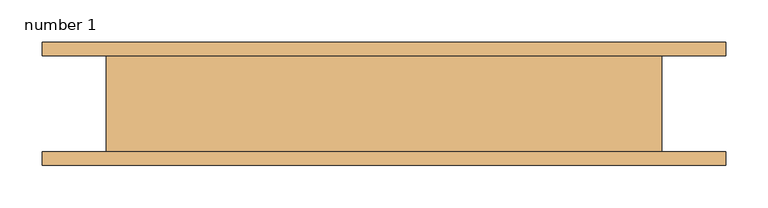
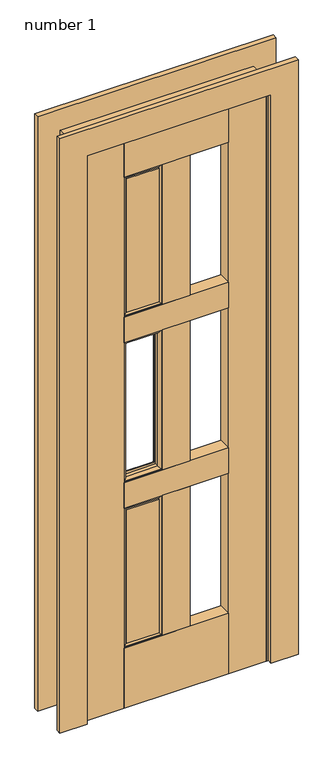
"""IFC4 building model written with IfcOpenShell, lengths in millimetres: door geometry, Door-Interior-Karona-K5660-6_Panel : number 1."""

from ifc_helpers import new_model, si_unit, frame, origin, origin_with_axes, place, context, project, spatial, polyline, ellipse_curve, outline, extrude, faceted_brep, source, transform, mapped, element, save
from ifc_brep_helpers import plane_surface, cylinder_surface, revolved_surface, advanced_brep


def number_1_f33ada90(model_context):
    return source(origin(), model_context, "Body", "SolidModel", [
        advanced_brep(
        [(-177.8, -15.2908, 1311.275), (-46.0375, -15.2908, 1311.275), (-57.3628137, -24.6126, 1299.9496863), (-166.4746863, -24.6126, 1299.9496863), (-57.1627, -46.3324899, 1300.1498), (-57.1627, -46.3324899, 820.7502), (-48.2727, -54.4576, 811.8602), (-48.2727, -54.4576, 1309.0398), (-166.6748, -46.3324899, 820.7502), (-166.6748, -46.3324899, 1300.1498), (-175.5648, -54.4576, 1309.0398), (-175.5648, -54.4576, 811.8602), (-46.0375, -54.4576, 809.625), (-177.8, -54.4576, 809.625), (-177.8, -15.2908, 809.625), (-46.0375, -15.2908, 809.625), (-57.1627, -34.7218, 820.7502), (-166.6748, -34.7218, 820.7502), (-47.3075, -24.6126, 1310.005), (-47.3075, -24.6126, 810.895), (-47.3075, -34.7218, 810.895), (-47.3075, -34.7218, 1310.005), (-176.53, -24.6126, 810.895), (-176.53, -24.6126, 1310.005), (-57.3628137, -24.6126, 820.9503137), (-166.4746863, -24.6126, 820.9503137), (-176.53, -34.7218, 810.895), (-177.8, -54.4576, 1311.275), (-166.6748, -34.7218, 1300.1498), (-176.53, -34.7218, 1310.005), (-46.0375, -54.4576, 1311.275), (-57.1627, -34.7218, 1300.1498)],
        [
            (0, 1),
            (1, 2, ellipse_curve(frame((-47.0685124, -25.5788135, 1310.2439876), z_axis=(-0.7071067811865475, 0.0, 0.7071067811865475), x_axis=(-0.7071067811865476, 0.0, -0.7071067811865474)), 14.6223259, 10.3395458)),
            (2, 3),
            (3, 0, ellipse_curve(frame((-176.7689876, -25.5788135, 1310.2439876), z_axis=(0.7071067811865475, 0.0, 0.7071067811865475), x_axis=(-0.7071067811865476, 0.0, 0.7071067811865474)), 14.6223259, 10.3395458)),
            (4, 5),
            (5, 6, ellipse_curve(frame((-48.2727, -45.531597, 811.8602), z_axis=(0.7071067811865475, 0.0, 0.7071067811865475), x_axis=(-0.7071067811865474, 0.0, 0.7071067811865476)), 12.6232745, 8.926003)),
            (6, 7),
            (7, 4, ellipse_curve(frame((-48.2727, -45.531597, 1309.0398), z_axis=(0.7071067811865475, 0.0, -0.7071067811865475), x_axis=(0.7071067811865474, 0.0, 0.7071067811865476)), 12.6232745, 8.926003)),
            (8, 9),
            (9, 10, ellipse_curve(frame((-175.5648, -45.531597, 1309.0398), z_axis=(-0.7071067811865475, 0.0, -0.7071067811865475), x_axis=(0.7071067811865474, 0.0, -0.7071067811865476)), 12.6232745, 8.926003)),
            (10, 11),
            (11, 8, ellipse_curve(frame((-175.5648, -45.531597, 811.8602), z_axis=(-0.7071067811865475, 0.0, 0.7071067811865475), x_axis=(-0.7071067811865474, 0.0, -0.7071067811865476)), 12.6232745, 8.926003)),
            (12, 13),
            (13, 14),
            (14, 15),
            (15, 12),
            (16, 17),
            (17, 8),
            (8, 5),
            (5, 16),
            (18, 19),
            (19, 20),
            (20, 21),
            (21, 18),
            (22, 19),
            (18, 23),
            (23, 22),
            (24, 25),
            (25, 3),
            (2, 24),
            (14, 25, ellipse_curve(frame((-176.7689876, -25.5788135, 810.6560124), z_axis=(0.7071067811865475, 0.0, -0.7071067811865475), x_axis=(0.7071067811865476, 0.0, 0.7071067811865474)), 14.6223259, 10.3395458)),
            (24, 15, ellipse_curve(frame((-47.0685124, -25.5788135, 810.6560124), z_axis=(-0.7071067811865475, 0.0, -0.7071067811865475), x_axis=(0.7071067811865476, 0.0, -0.7071067811865474)), 14.6223259, 10.3395458)),
            (22, 26),
            (26, 20),
            (13, 27),
            (27, 0),
            (0, 14),
            (17, 28),
            (28, 9),
            (23, 29),
            (29, 26),
            (27, 30),
            (30, 1),
            (28, 31),
            (31, 4),
            (4, 9),
            (21, 29),
            (30, 12),
            (15, 1),
            (31, 16),
            (6, 11),
            (10, 7),
        ],
        [
            cylinder_surface(frame((-177.8, -25.5788135, 1310.2439876), z_axis=(-1.0, 0.0, 0.0), x_axis=(0.0, 1.0, 0.0)), 10.3395458),
            cylinder_surface(frame((-48.2727, -45.531597, 1311.275), z_axis=(0.0, 0.0, 1.0), x_axis=(0.0, 1.0, 0.0)), 8.926003),
            cylinder_surface(frame((-175.5648, -45.531597, 809.625), z_axis=(0.0, 0.0, -1.0), x_axis=(0.0, 1.0, 0.0)), 8.926003),
            plane_surface(frame((-46.0375, -15.2908, 809.625), z_axis=(0.0, 0.0, -1.0), x_axis=(-1.0, 0.0, 0.0))),
            plane_surface(frame((-57.1627, -46.3324899, 820.7502), z_axis=(0.0, 0.0, 1.0), x_axis=(-1.0, 0.0, 0.0))),
            plane_surface(frame((-47.3075, -34.7218, 1310.005), z_axis=(-1.0, 0.0, 0.0), x_axis=(0.0, 0.0, -1.0))),
            plane_surface(frame((-47.3075, -24.6126, 1310.005), z_axis=(0.0, -1.0, 0.0), x_axis=(0.0, 0.0, -1.0))),
            cylinder_surface(frame((-46.0375, -25.5788135, 810.6560124), z_axis=(1.0, 0.0, 0.0), x_axis=(0.0, 1.0, 0.0)), 10.3395458),
            plane_surface(frame((-47.3075, -34.7218, 810.895), z_axis=(0.0, 0.0, 1.0), x_axis=(-1.0, 0.0, 0.0))),
            plane_surface(frame((-177.8, -15.2908, 809.625), z_axis=(-1.0, 0.0, 0.0), x_axis=(0.0, 0.0, 1.0))),
            plane_surface(frame((-166.6748, -46.3324899, 820.7502), z_axis=(1.0, 0.0, 0.0), x_axis=(0.0, 0.0, 1.0))),
            plane_surface(frame((-176.53, -34.7218, 810.895), z_axis=(1.0, 0.0, 0.0), x_axis=(0.0, 0.0, 1.0))),
            plane_surface(frame((-177.8, -15.2908, 1311.275), z_axis=(0.0, 0.0, 1.0), x_axis=(1.0, 0.0, 0.0))),
            plane_surface(frame((-166.6748, -46.3324899, 1300.1498), z_axis=(0.0, 0.0, -1.0), x_axis=(1.0, 0.0, 0.0))),
            plane_surface(frame((-176.53, -34.7218, 1310.005), z_axis=(0.0, 0.0, -1.0), x_axis=(1.0, 0.0, 0.0))),
            plane_surface(frame((-46.0375, -15.2908, 1311.275), z_axis=(1.0, 0.0, 0.0), x_axis=(0.0, 0.0, -1.0))),
            plane_surface(frame((-57.1627, -46.3324899, 1300.1498), z_axis=(-1.0, 0.0, 0.0), x_axis=(0.0, 0.0, -1.0))),
            plane_surface(frame((-57.1627, -34.7218, 1300.1498), z_axis=(0.0, 1.0, 0.0), x_axis=(0.0, 0.0, -1.0))),
            plane_surface(frame((-46.0375, -54.4576, 1311.275), z_axis=(0.0, -1.0, 0.0), x_axis=(0.0, 0.0, -1.0))),
            cylinder_surface(frame((-46.0375, -45.531597, 811.8602), z_axis=(1.0, 0.0, 0.0), x_axis=(0.0, 1.0, 0.0)), 8.926003),
            cylinder_surface(frame((-176.7689876, -25.5788135, 809.625), z_axis=(0.0, 0.0, -1.0), x_axis=(0.0, 1.0, 0.0)), 10.3395458),
            cylinder_surface(frame((-177.8, -45.531597, 1309.0398), z_axis=(-1.0, 0.0, 0.0), x_axis=(0.0, 1.0, 0.0)), 8.926003),
            cylinder_surface(frame((-47.0685124, -25.5788135, 1311.275), z_axis=(0.0, 0.0, 1.0), x_axis=(0.0, 1.0, 0.0)), 10.3395458),
        ],
        [
            (0, [[1, 2, 3, 4]]),
            (1, [[5, 6, 7, 8]]),
            (2, [[9, 10, 11, 12]]),
            (3, [[13, 14, 15, 16]]),
            (4, [[17, 18, 19, 20]]),
            (5, [[21, 22, 23, 24]]),
            (6, [[25, -21, 26, 27], [28, 29, -3, 30]]),
            (7, [[-15, 31, -28, 32]]),
            (8, [[-25, 33, 34, -22]]),
            (9, [[35, 36, 37, -14]]),
            (10, [[38, 39, -9, -18]]),
            (11, [[-27, 40, 41, -33]]),
            (12, [[42, 43, -1, -36]]),
            (13, [[44, 45, 46, -39]]),
            (14, [[-26, -24, 47, -40]]),
            (15, [[48, -16, 49, -43]]),
            (16, [[50, -20, -5, -45]]),
            (17, [[-34, -41, -47, -23], [-17, -50, -44, -38]]),
            (18, [[-13, -48, -42, -35], [51, -11, 52, -7]]),
            (19, [[-19, -12, -51, -6]]),
            (20, [[-37, -4, -29, -31]]),
            (21, [[-46, -8, -52, -10]]),
            (22, [[-49, -32, -30, -2]]),
        ],
    ),
        advanced_brep(
        [(-166.6748, -54.4576, 1893.8748), (-166.6748, -54.4576, 1414.4752), (-57.1627, -54.4576, 1414.4752), (-57.1627, -54.4576, 1893.8748), (-166.6748, -34.7218, 1893.8748), (-166.6748, -36.0454899, 1893.8748), (-57.1627, -36.0454899, 1893.8748), (-57.1627, -34.7218, 1893.8748), (-57.1627, -44.5515929, 1893.8748), (-166.6748, -44.5515929, 1893.8748), (-57.1627, -34.7218, 1414.4752), (-57.1627, -36.0454899, 1414.4752), (-166.6748, -36.0454899, 1414.4752), (-166.6748, -34.7218, 1414.4752), (-166.6748, -44.5515929, 1414.4752), (-57.1627, -44.5515929, 1414.4752), (-87.1686653, -44.5515929, 1863.8688347), (-136.6688347, -44.5515929, 1863.8688347), (-87.1686653, -44.5515929, 1444.4811653), (-136.6688347, -44.5515929, 1444.4811653)],
        [
            (0, 1),
            (1, 2),
            (2, 3),
            (3, 0),
            (4, 5),
            (5, 6),
            (6, 7),
            (7, 4),
            (3, 8),
            (8, 9),
            (9, 0),
            (10, 11),
            (11, 12),
            (12, 13),
            (13, 10),
            (1, 14),
            (14, 15),
            (15, 2),
            (9, 14),
            (12, 5),
            (4, 13),
            (6, 11),
            (10, 7),
            (15, 8),
            (16, 6, ellipse_curve(frame((-55.2243315, -100.0605261, 1895.8131685), z_axis=(0.7071067811865475, 0.0, -0.7071067811865475), x_axis=(-0.7071067811865476, 0.0, -0.7071067811865474)), 90.5724254, 64.0443762)),
            (5, 17, ellipse_curve(frame((-168.6131685, -100.0605261, 1895.8131685), z_axis=(-0.7071067811865475, 0.0, -0.7071067811865475), x_axis=(-0.7071067811865476, 0.0, 0.7071067811865474)), 90.5724254, 64.0443762)),
            (17, 16),
            (18, 11, ellipse_curve(frame((-55.2243315, -100.0605261, 1412.5368315), z_axis=(-0.7071067811865475, 0.0, -0.7071067811865475), x_axis=(-0.7071067811865474, 0.0, 0.7071067811865476)), 90.5724254, 64.0443762)),
            (16, 18),
            (19, 12, ellipse_curve(frame((-168.6131685, -100.0605261, 1412.5368315), z_axis=(-0.7071067811865475, 0.0, 0.7071067811865475), x_axis=(0.7071067811865476, 0.0, 0.7071067811865474)), 90.5724254, 64.0443762)),
            (18, 19),
            (19, 17),
        ],
        [
            plane_surface(frame((-57.1627, -54.4576, 1893.8748), z_axis=(0.0, -1.0, 0.0), x_axis=(0.0, 0.0, -1.0))),
            plane_surface(frame((-57.1627, -34.7218, 1893.8748), z_axis=(0.0, 0.0, 1.0), x_axis=(1.0, 0.0, 0.0))),
            plane_surface(frame((-57.1627, -34.7218, 1414.4752), z_axis=(0.0, 0.0, -1.0), x_axis=(-1.0, 0.0, 0.0))),
            plane_surface(frame((-166.6748, -54.4576, 1893.8748), z_axis=(-1.0, 0.0, 0.0), x_axis=(0.0, 0.0, -1.0))),
            plane_surface(frame((-57.1627, -34.7218, 1893.8748), z_axis=(1.0, 0.0, 0.0), x_axis=(0.0, 0.0, -1.0))),
            plane_surface(frame((-166.6748, -34.7218, 1893.8748), z_axis=(0.0, 1.0, 0.0), x_axis=(0.0, 0.0, -1.0))),
            revolved_surface(polyline([(-232.6575446888527, -100.0605261, 1831.7687923), (8.820044688852704, -100.0605261, 1831.7687923)]), (-177.8, -100.0605261, 1895.8131685), (-1.0, 0.0, 0.0)),
            revolved_surface(polyline([(-119.2687077, -100.0605261, 1959.8575446888528), (-119.2687077, -100.0605261, 1348.4924553111473)]), (-55.2243315, -100.0605261, 1905.0), (0.0, 0.0, 1.0)),
            revolved_surface(polyline([(8.820044688852683, -100.0605261, 1476.5812077), (-232.6575446888527, -100.0605261, 1476.5812077)]), (-46.0375, -100.0605261, 1412.5368315), (1.0, 0.0, 0.0)),
            revolved_surface(polyline([(-104.5687923, -100.0605261, 1348.4924553111473), (-104.5687923, -100.0605261, 1959.8575446888526)]), (-168.6131685, -100.0605261, 1403.35), (0.0, 0.0, -1.0)),
            plane_surface(frame((-177.8, -44.5515929, 1403.35), z_axis=(0.0, 1.0, 0.0), x_axis=(0.0, 0.0, 1.0))),
        ],
        [
            (0, [[1, 2, 3, 4]]),
            (1, [[5, 6, 7, 8]]),
            (1, [[9, 10, 11, -4]]),
            (2, [[12, 13, 14, 15]]),
            (2, [[16, 17, 18, -2]]),
            (3, [[-11, 19, -16, -1]]),
            (3, [[-14, 20, -5, 21]]),
            (4, [[-7, 22, -12, 23]]),
            (4, [[-18, 24, -9, -3]]),
            (5, [[-23, -15, -21, -8]]),
            (6, [[25, -6, 26, 27]]),
            (7, [[28, -22, -25, 29]]),
            (8, [[30, -13, -28, 31]]),
            (9, [[-26, -20, -30, 32]]),
            (10, [[-24, -17, -19, -10], [-32, -31, -29, -27]]),
        ],
    ),
        advanced_brep(
        [(-166.6748, -24.6126, 1893.8748), (-166.6748, -24.6126, 1414.4752), (-57.1627, -24.6126, 1414.4752), (-57.1627, -24.6126, 1893.8748), (-137.8448579, -15.4432, 1443.3051421), (-137.8448579, -15.4432, 1865.0448579), (-85.9926421, -15.4432, 1865.0448579), (-85.9926421, -15.4432, 1443.3051421), (-57.1627, -23.2889101, 1893.8748), (-166.6748, -23.2889101, 1893.8748), (-166.6748, -23.2889101, 1414.4752), (-57.1627, -23.2889101, 1414.4752)],
        [
            (0, 1),
            (1, 2),
            (2, 3),
            (3, 0),
            (4, 5),
            (5, 6),
            (6, 7),
            (7, 4),
            (3, 8),
            (8, 9),
            (9, 0),
            (1, 10),
            (10, 11),
            (11, 2),
            (7, 11, ellipse_curve(frame((-55.2243315, 40.7261261, 1412.5368315), z_axis=(0.7071067811865475, 0.0, 0.7071067811865475), x_axis=(0.7071067811865476, 0.0, -0.7071067811865474)), 90.5724254, 64.0443762)),
            (10, 4, ellipse_curve(frame((-168.6131685, 40.7261261, 1412.5368315), z_axis=(-0.7071067811865475, 0.0, 0.7071067811865475), x_axis=(0.7071067811865476, 0.0, 0.7071067811865474)), 90.5724254, 64.0443762)),
            (10, 9),
            (9, 5, ellipse_curve(frame((-168.6131685, 40.7261261, 1895.8131685), z_axis=(0.7071067811865475, 0.0, 0.7071067811865475), x_axis=(0.7071067811865474, 0.0, -0.7071067811865476)), 90.5724254, 64.0443762)),
            (8, 6, ellipse_curve(frame((-55.2243315, 40.7261261, 1895.8131685), z_axis=(0.7071067811865475, 0.0, -0.7071067811865475), x_axis=(-0.7071067811865476, 0.0, -0.7071067811865474)), 90.5724254, 64.0443762)),
            (8, 11),
        ],
        [
            plane_surface(frame((-57.1627, -24.6126, 1893.8748), z_axis=(0.0, -1.0, 0.0), x_axis=(0.0, 0.0, -1.0))),
            plane_surface(frame((-166.6748, -15.4432, 1893.8748), z_axis=(0.0, 1.0, 0.0), x_axis=(0.0, 0.0, -1.0))),
            plane_surface(frame((-57.1627, -34.7218, 1893.8748), z_axis=(0.0, 0.0, 1.0), x_axis=(1.0, 0.0, 0.0))),
            plane_surface(frame((-57.1627, -34.7218, 1414.4752), z_axis=(0.0, 0.0, -1.0), x_axis=(-1.0, 0.0, 0.0))),
            revolved_surface(polyline([(8.820044688852711, 40.7261261, 1476.5812077), (-232.6575446888527, 40.7261261, 1476.5812077)]), (-46.0375, 40.7261261, 1412.5368315), (1.0, 0.0, 0.0)),
            revolved_surface(polyline([(-104.5687923, 40.7261261, 1348.4924553111473), (-104.5687923, 40.7261261, 1959.8575446888528)]), (-168.6131685, 40.7261261, 1403.35), (0.0, 0.0, -1.0)),
            revolved_surface(polyline([(-232.65754468885268, 40.7261261, 1831.7687923), (8.820044688852704, 40.7261261, 1831.7687923)]), (-177.8, 40.7261261, 1895.8131685), (-1.0, 0.0, 0.0)),
            revolved_surface(polyline([(-119.2687077, 40.7261261, 1959.8575446888528), (-119.2687077, 40.7261261, 1348.4924553111473)]), (-55.2243315, 40.7261261, 1905.0), (0.0, 0.0, 1.0)),
            plane_surface(frame((-166.6748, -24.6126, 1893.8748), z_axis=(-1.0, 0.0, 0.0), x_axis=(0.0, 0.0, -1.0))),
            plane_surface(frame((-57.1627, -15.4432, 1893.8748), z_axis=(1.0, 0.0, 0.0), x_axis=(0.0, 0.0, -1.0))),
        ],
        [
            (0, [[1, 2, 3, 4]]),
            (1, [[5, 6, 7, 8]]),
            (2, [[9, 10, 11, -4]]),
            (3, [[12, 13, 14, -2]]),
            (4, [[-8, 15, -13, 16]]),
            (5, [[17, 18, -5, -16]]),
            (6, [[-10, 19, -6, -18]]),
            (7, [[20, -15, -7, -19]]),
            (8, [[-11, -17, -12, -1]]),
            (9, [[-14, -20, -9, -3]]),
        ],
    ),
        advanced_brep(
        [(-177.8, -15.2908, 1905.0), (-46.0375, -15.2908, 1905.0), (-57.3628137, -24.6126, 1893.6746863), (-166.4746863, -24.6126, 1893.6746863), (-57.1627, -46.3324899, 1893.8748), (-57.1627, -46.3324899, 1414.4752), (-48.2727, -54.4576, 1405.5852), (-48.2727, -54.4576, 1902.7648), (-166.6748, -46.3324899, 1414.4752), (-166.6748, -46.3324899, 1893.8748), (-175.5648, -54.4576, 1902.7648), (-175.5648, -54.4576, 1405.5852), (-46.0375, -54.4576, 1403.35), (-177.8, -54.4576, 1403.35), (-177.8, -15.2908, 1403.35), (-46.0375, -15.2908, 1403.35), (-57.1627, -34.7218, 1414.4752), (-166.6748, -34.7218, 1414.4752), (-47.3075, -24.6126, 1903.73), (-47.3075, -24.6126, 1404.62), (-47.3075, -34.7218, 1404.62), (-47.3075, -34.7218, 1903.73), (-176.53, -24.6126, 1404.62), (-176.53, -24.6126, 1903.73), (-57.3628137, -24.6126, 1414.6753137), (-166.4746863, -24.6126, 1414.6753137), (-176.53, -34.7218, 1404.62), (-177.8, -54.4576, 1905.0), (-166.6748, -34.7218, 1893.8748), (-176.53, -34.7218, 1903.73), (-46.0375, -54.4576, 1905.0), (-57.1627, -34.7218, 1893.8748)],
        [
            (0, 1),
            (1, 2, ellipse_curve(frame((-47.0685124, -25.5788135, 1903.9689876), z_axis=(-0.7071067811865475, 0.0, 0.7071067811865475), x_axis=(-0.7071067811865476, 0.0, -0.7071067811865474)), 14.6223259, 10.3395458)),
            (2, 3),
            (3, 0, ellipse_curve(frame((-176.7689876, -25.5788135, 1903.9689876), z_axis=(0.7071067811865475, 0.0, 0.7071067811865475), x_axis=(-0.7071067811865476, 0.0, 0.7071067811865474)), 14.6223259, 10.3395458)),
            (4, 5),
            (5, 6, ellipse_curve(frame((-48.2727, -45.531597, 1405.5852), z_axis=(0.7071067811865475, 0.0, 0.7071067811865475), x_axis=(-0.7071067811865474, 0.0, 0.7071067811865476)), 12.6232745, 8.926003)),
            (6, 7),
            (7, 4, ellipse_curve(frame((-48.2727, -45.531597, 1902.7648), z_axis=(0.7071067811865475, 0.0, -0.7071067811865475), x_axis=(0.7071067811865474, 0.0, 0.7071067811865476)), 12.6232745, 8.926003)),
            (8, 9),
            (9, 10, ellipse_curve(frame((-175.5648, -45.531597, 1902.7648), z_axis=(-0.7071067811865475, 0.0, -0.7071067811865475), x_axis=(0.7071067811865474, 0.0, -0.7071067811865476)), 12.6232745, 8.926003)),
            (10, 11),
            (11, 8, ellipse_curve(frame((-175.5648, -45.531597, 1405.5852), z_axis=(-0.7071067811865475, 0.0, 0.7071067811865475), x_axis=(-0.7071067811865474, 0.0, -0.7071067811865476)), 12.6232745, 8.926003)),
            (12, 13),
            (13, 14),
            (14, 15),
            (15, 12),
            (16, 17),
            (17, 8),
            (8, 5),
            (5, 16),
            (18, 19),
            (19, 20),
            (20, 21),
            (21, 18),
            (22, 19),
            (18, 23),
            (23, 22),
            (24, 25),
            (25, 3),
            (2, 24),
            (14, 25, ellipse_curve(frame((-176.7689876, -25.5788135, 1404.3810124), z_axis=(0.7071067811865475, 0.0, -0.7071067811865475), x_axis=(0.7071067811865476, 0.0, 0.7071067811865474)), 14.6223259, 10.3395458)),
            (24, 15, ellipse_curve(frame((-47.0685124, -25.5788135, 1404.3810124), z_axis=(-0.7071067811865475, 0.0, -0.7071067811865475), x_axis=(0.7071067811865476, 0.0, -0.7071067811865474)), 14.6223259, 10.3395458)),
            (22, 26),
            (26, 20),
            (13, 27),
            (27, 0),
            (0, 14),
            (17, 28),
            (28, 9),
            (23, 29),
            (29, 26),
            (27, 30),
            (30, 1),
            (28, 31),
            (31, 4),
            (4, 9),
            (21, 29),
            (30, 12),
            (15, 1),
            (31, 16),
            (6, 11),
            (10, 7),
        ],
        [
            cylinder_surface(frame((-177.8, -25.5788135, 1903.9689876), z_axis=(-1.0, 0.0, 0.0), x_axis=(0.0, 1.0, 0.0)), 10.3395458),
            cylinder_surface(frame((-48.2727, -45.531597, 1905.0), z_axis=(0.0, 0.0, 1.0), x_axis=(0.0, 1.0, 0.0)), 8.926003),
            cylinder_surface(frame((-175.5648, -45.531597, 1403.35), z_axis=(0.0, 0.0, -1.0), x_axis=(0.0, 1.0, 0.0)), 8.926003),
            plane_surface(frame((-46.0375, -15.2908, 1403.35), z_axis=(0.0, 0.0, -1.0), x_axis=(-1.0, 0.0, 0.0))),
            plane_surface(frame((-57.1627, -46.3324899, 1414.4752), z_axis=(0.0, 0.0, 1.0), x_axis=(-1.0, 0.0, 0.0))),
            plane_surface(frame((-47.3075, -34.7218, 1903.73), z_axis=(-1.0, 0.0, 0.0), x_axis=(0.0, 0.0, -1.0))),
            plane_surface(frame((-47.3075, -24.6126, 1903.73), z_axis=(0.0, -1.0, 0.0), x_axis=(0.0, 0.0, -1.0))),
            cylinder_surface(frame((-46.0375, -25.5788135, 1404.3810124), z_axis=(1.0, 0.0, 0.0), x_axis=(0.0, 1.0, 0.0)), 10.3395458),
            plane_surface(frame((-47.3075, -34.7218, 1404.62), z_axis=(0.0, 0.0, 1.0), x_axis=(-1.0, 0.0, 0.0))),
            plane_surface(frame((-177.8, -15.2908, 1403.35), z_axis=(-1.0, 0.0, 0.0), x_axis=(0.0, 0.0, 1.0))),
            plane_surface(frame((-166.6748, -46.3324899, 1414.4752), z_axis=(1.0, 0.0, 0.0), x_axis=(0.0, 0.0, 1.0))),
            plane_surface(frame((-176.53, -34.7218, 1404.62), z_axis=(1.0, 0.0, 0.0), x_axis=(0.0, 0.0, 1.0))),
            plane_surface(frame((-177.8, -15.2908, 1905.0), z_axis=(0.0, 0.0, 1.0), x_axis=(1.0, 0.0, 0.0))),
            plane_surface(frame((-166.6748, -46.3324899, 1893.8748), z_axis=(0.0, 0.0, -1.0), x_axis=(1.0, 0.0, 0.0))),
            plane_surface(frame((-176.53, -34.7218, 1903.73), z_axis=(0.0, 0.0, -1.0), x_axis=(1.0, 0.0, 0.0))),
            plane_surface(frame((-46.0375, -15.2908, 1905.0), z_axis=(1.0, 0.0, 0.0), x_axis=(0.0, 0.0, -1.0))),
            plane_surface(frame((-57.1627, -46.3324899, 1893.8748), z_axis=(-1.0, 0.0, 0.0), x_axis=(0.0, 0.0, -1.0))),
            plane_surface(frame((-57.1627, -34.7218, 1893.8748), z_axis=(0.0, 1.0, 0.0), x_axis=(0.0, 0.0, -1.0))),
            plane_surface(frame((-46.0375, -54.4576, 1905.0), z_axis=(0.0, -1.0, 0.0), x_axis=(0.0, 0.0, -1.0))),
            cylinder_surface(frame((-46.0375, -45.531597, 1405.5852), z_axis=(1.0, 0.0, 0.0), x_axis=(0.0, 1.0, 0.0)), 8.926003),
            cylinder_surface(frame((-176.7689876, -25.5788135, 1403.35), z_axis=(0.0, 0.0, -1.0), x_axis=(0.0, 1.0, 0.0)), 10.3395458),
            cylinder_surface(frame((-177.8, -45.531597, 1902.7648), z_axis=(-1.0, 0.0, 0.0), x_axis=(0.0, 1.0, 0.0)), 8.926003),
            cylinder_surface(frame((-47.0685124, -25.5788135, 1905.0), z_axis=(0.0, 0.0, 1.0), x_axis=(0.0, 1.0, 0.0)), 10.3395458),
        ],
        [
            (0, [[1, 2, 3, 4]]),
            (1, [[5, 6, 7, 8]]),
            (2, [[9, 10, 11, 12]]),
            (3, [[13, 14, 15, 16]]),
            (4, [[17, 18, 19, 20]]),
            (5, [[21, 22, 23, 24]]),
            (6, [[25, -21, 26, 27], [28, 29, -3, 30]]),
            (7, [[-15, 31, -28, 32]]),
            (8, [[-25, 33, 34, -22]]),
            (9, [[35, 36, 37, -14]]),
            (10, [[38, 39, -9, -18]]),
            (11, [[-27, 40, 41, -33]]),
            (12, [[42, 43, -1, -36]]),
            (13, [[44, 45, 46, -39]]),
            (14, [[-26, -24, 47, -40]]),
            (15, [[48, -16, 49, -43]]),
            (16, [[50, -20, -5, -45]]),
            (17, [[-34, -41, -47, -23], [-17, -50, -44, -38]]),
            (18, [[-13, -48, -42, -35], [51, -11, 52, -7]]),
            (19, [[-19, -12, -51, -6]]),
            (20, [[-37, -4, -29, -31]]),
            (21, [[-46, -8, -52, -10]]),
            (22, [[-49, -32, -30, -2]]),
        ],
    ),
        advanced_brep(
        [(-166.6748, -34.7218, 706.4248), (-166.6748, -36.0454899, 706.4248), (-57.1627, -36.0454899, 706.4248), (-57.1627, -34.7218, 706.4248), (-57.1627, -54.4576, 706.4248), (-57.1627, -44.5515929, 706.4248), (-166.6748, -44.5515929, 706.4248), (-166.6748, -54.4576, 706.4248), (-57.1627, -34.7218, 227.0252), (-57.1627, -36.0454899, 227.0252), (-166.6748, -36.0454899, 227.0252), (-166.6748, -34.7218, 227.0252), (-166.6748, -54.4576, 227.0252), (-166.6748, -44.5515929, 227.0252), (-57.1627, -44.5515929, 227.0252), (-57.1627, -54.4576, 227.0252), (-87.1686653, -44.5515929, 676.4188347), (-136.6688347, -44.5515929, 676.4188347), (-87.1686653, -44.5515929, 257.0311653), (-136.6688347, -44.5515929, 257.0311653)],
        [
            (0, 1),
            (1, 2),
            (2, 3),
            (3, 0),
            (4, 5),
            (5, 6),
            (6, 7),
            (7, 4),
            (8, 9),
            (9, 10),
            (10, 11),
            (11, 8),
            (12, 13),
            (13, 14),
            (14, 15),
            (15, 12),
            (6, 13),
            (12, 7),
            (10, 1),
            (0, 11),
            (15, 4),
            (2, 9),
            (8, 3),
            (14, 5),
            (16, 2, ellipse_curve(frame((-55.2243315, -100.0605261, 708.3631685), z_axis=(0.7071067811865475, 0.0, -0.7071067811865475), x_axis=(-0.7071067811865476, 0.0, -0.7071067811865474)), 90.5724254, 64.0443762)),
            (1, 17, ellipse_curve(frame((-168.6131685, -100.0605261, 708.3631685), z_axis=(-0.7071067811865475, 0.0, -0.7071067811865475), x_axis=(-0.7071067811865476, 0.0, 0.7071067811865474)), 90.5724254, 64.0443762)),
            (17, 16),
            (18, 9, ellipse_curve(frame((-55.2243315, -100.0605261, 225.0868315), z_axis=(-0.7071067811865475, 0.0, -0.7071067811865475), x_axis=(-0.7071067811865474, 0.0, 0.7071067811865476)), 90.5724254, 64.0443762)),
            (16, 18),
            (19, 10, ellipse_curve(frame((-168.6131685, -100.0605261, 225.0868315), z_axis=(-0.7071067811865475, 0.0, 0.7071067811865475), x_axis=(0.7071067811865476, 0.0, 0.7071067811865474)), 90.5724254, 64.0443762)),
            (18, 19),
            (19, 17),
        ],
        [
            plane_surface(frame((-57.1627, -34.7218, 706.4248), z_axis=(0.0, 0.0, 1.0), x_axis=(1.0, 0.0, 0.0))),
            plane_surface(frame((-57.1627, -34.7218, 227.0252), z_axis=(0.0, 0.0, -1.0), x_axis=(-1.0, 0.0, 0.0))),
            plane_surface(frame((-166.6748, -54.4576, 706.4248), z_axis=(-1.0, 0.0, 0.0), x_axis=(0.0, 0.0, -1.0))),
            plane_surface(frame((-57.1627, -54.4576, 706.4248), z_axis=(0.0, -1.0, 0.0), x_axis=(0.0, 0.0, -1.0))),
            plane_surface(frame((-57.1627, -34.7218, 706.4248), z_axis=(1.0, 0.0, 0.0), x_axis=(0.0, 0.0, -1.0))),
            plane_surface(frame((-166.6748, -34.7218, 706.4248), z_axis=(0.0, 1.0, 0.0), x_axis=(0.0, 0.0, -1.0))),
            revolved_surface(polyline([(-232.6575446888527, -100.0605261, 644.3187923), (8.820044688852704, -100.0605261, 644.3187923)]), (-177.8, -100.0605261, 708.3631685), (-1.0, 0.0, 0.0)),
            revolved_surface(polyline([(-119.2687077, -100.0605261, 772.4075446888527), (-119.2687077, -100.0605261, 161.04245531114725)]), (-55.2243315, -100.0605261, 717.55), (0.0, 0.0, 1.0)),
            revolved_surface(polyline([(8.820044688852683, -100.0605261, 289.1312077), (-232.6575446888527, -100.0605261, 289.1312077)]), (-46.0375, -100.0605261, 225.0868315), (1.0, 0.0, 0.0)),
            revolved_surface(polyline([(-104.5687923, -100.0605261, 161.0424553111473), (-104.5687923, -100.0605261, 772.4075446888527)]), (-168.6131685, -100.0605261, 215.9), (0.0, 0.0, -1.0)),
            plane_surface(frame((-177.8, -44.5515929, 215.9), z_axis=(0.0, 1.0, 0.0), x_axis=(0.0, 0.0, 1.0))),
        ],
        [
            (0, [[1, 2, 3, 4]]),
            (0, [[5, 6, 7, 8]]),
            (1, [[9, 10, 11, 12]]),
            (1, [[13, 14, 15, 16]]),
            (2, [[-7, 17, -13, 18]]),
            (2, [[-11, 19, -1, 20]]),
            (3, [[-18, -16, 21, -8]]),
            (4, [[-3, 22, -9, 23]]),
            (4, [[-15, 24, -5, -21]]),
            (5, [[-23, -12, -20, -4]]),
            (6, [[25, -2, 26, 27]]),
            (7, [[28, -22, -25, 29]]),
            (8, [[30, -10, -28, 31]]),
            (9, [[-26, -19, -30, 32]]),
            (10, [[-24, -14, -17, -6], [-32, -31, -29, -27]]),
        ],
    ),
        advanced_brep(
        [(-57.1627, -24.6126, 706.4248), (-57.1627, -23.2889101, 706.4248), (-166.6748, -23.2889101, 706.4248), (-166.6748, -24.6126, 706.4248), (-166.6748, -24.6126, 227.0252), (-166.6748, -23.2889101, 227.0252), (-57.1627, -23.2889101, 227.0252), (-57.1627, -24.6126, 227.0252), (-137.8448579, -15.4432, 255.8551421), (-137.8448579, -15.4432, 677.5948579), (-85.9926421, -15.4432, 677.5948579), (-85.9926421, -15.4432, 255.8551421)],
        [
            (0, 1),
            (1, 2),
            (2, 3),
            (3, 0),
            (4, 5),
            (5, 6),
            (6, 7),
            (7, 4),
            (3, 4),
            (7, 0),
            (8, 9),
            (9, 10),
            (10, 11),
            (11, 8),
            (11, 6, ellipse_curve(frame((-55.2243315, 40.7261261, 225.0868315), z_axis=(0.7071067811865475, 0.0, 0.7071067811865475), x_axis=(0.7071067811865476, 0.0, -0.7071067811865474)), 90.5724254, 64.0443762)),
            (5, 8, ellipse_curve(frame((-168.6131685, 40.7261261, 225.0868315), z_axis=(-0.7071067811865475, 0.0, 0.7071067811865475), x_axis=(0.7071067811865476, 0.0, 0.7071067811865474)), 90.5724254, 64.0443762)),
            (5, 2),
            (2, 9, ellipse_curve(frame((-168.6131685, 40.7261261, 708.3631685), z_axis=(0.7071067811865475, 0.0, 0.7071067811865475), x_axis=(0.7071067811865474, 0.0, -0.7071067811865476)), 90.5724254, 64.0443762)),
            (1, 10, ellipse_curve(frame((-55.2243315, 40.7261261, 708.3631685), z_axis=(0.7071067811865475, 0.0, -0.7071067811865475), x_axis=(-0.7071067811865476, 0.0, -0.7071067811865474)), 90.5724254, 64.0443762)),
            (1, 6),
        ],
        [
            plane_surface(frame((-57.1627, -34.7218, 706.4248), z_axis=(0.0, 0.0, 1.0), x_axis=(1.0, 0.0, 0.0))),
            plane_surface(frame((-57.1627, -34.7218, 227.0252), z_axis=(0.0, 0.0, -1.0), x_axis=(-1.0, 0.0, 0.0))),
            plane_surface(frame((-57.1627, -24.6126, 706.4248), z_axis=(0.0, -1.0, 0.0), x_axis=(0.0, 0.0, -1.0))),
            plane_surface(frame((-166.6748, -15.4432, 706.4248), z_axis=(0.0, 1.0, 0.0), x_axis=(0.0, 0.0, -1.0))),
            revolved_surface(polyline([(8.820044688852711, 40.7261261, 289.1312077), (-232.6575446888527, 40.7261261, 289.1312077)]), (-46.0375, 40.7261261, 225.0868315), (1.0, 0.0, 0.0)),
            revolved_surface(polyline([(-104.5687923, 40.7261261, 161.0424553111473), (-104.5687923, 40.7261261, 772.4075446888527)]), (-168.6131685, 40.7261261, 215.9), (0.0, 0.0, -1.0)),
            revolved_surface(polyline([(-232.65754468885268, 40.7261261, 644.3187923), (8.820044688852704, 40.7261261, 644.3187923)]), (-177.8, 40.7261261, 708.3631685), (-1.0, 0.0, 0.0)),
            revolved_surface(polyline([(-119.2687077, 40.7261261, 772.4075446888527), (-119.2687077, 40.7261261, 161.04245531114736)]), (-55.2243315, 40.7261261, 717.55), (0.0, 0.0, 1.0)),
            plane_surface(frame((-166.6748, -24.6126, 706.4248), z_axis=(-1.0, 0.0, 0.0), x_axis=(0.0, 0.0, -1.0))),
            plane_surface(frame((-57.1627, -15.4432, 706.4248), z_axis=(1.0, 0.0, 0.0), x_axis=(0.0, 0.0, -1.0))),
        ],
        [
            (0, [[1, 2, 3, 4]]),
            (1, [[5, 6, 7, 8]]),
            (2, [[9, -8, 10, -4]]),
            (3, [[11, 12, 13, 14]]),
            (4, [[-14, 15, -6, 16]]),
            (5, [[17, 18, -11, -16]]),
            (6, [[-2, 19, -12, -18]]),
            (7, [[20, -15, -13, -19]]),
            (8, [[-3, -17, -5, -9]]),
            (9, [[-7, -20, -1, -10]]),
        ],
    ),
        advanced_brep(
        [(-177.8, -15.2908, 717.55), (-46.0375, -15.2908, 717.55), (-57.3628137, -24.6126, 706.2246863), (-166.4746863, -24.6126, 706.2246863), (-57.1627, -46.3324899, 706.4248), (-57.1627, -46.3324899, 227.0252), (-48.2727, -54.4576, 218.1352), (-48.2727, -54.4576, 715.3148), (-177.8, -54.4576, 215.9), (-46.0375, -54.4576, 215.9), (-46.0375, -54.4576, 717.55), (-177.8, -54.4576, 717.55), (-175.5648, -54.4576, 218.1352), (-175.5648, -54.4576, 715.3148), (-177.8, -15.2908, 215.9), (-46.0375, -15.2908, 215.9), (-57.1627, -34.7218, 227.0252), (-166.6748, -34.7218, 227.0252), (-166.6748, -46.3324899, 227.0252), (-47.3075, -24.6126, 217.17), (-176.53, -24.6126, 217.17), (-176.53, -34.7218, 217.17), (-47.3075, -34.7218, 217.17), (-166.6748, -34.7218, 706.4248), (-166.6748, -46.3324899, 706.4248), (-176.53, -24.6126, 716.28), (-176.53, -34.7218, 716.28), (-57.1627, -34.7218, 706.4248), (-47.3075, -24.6126, 716.28), (-47.3075, -34.7218, 716.28), (-57.3628137, -24.6126, 227.2253137), (-166.4746863, -24.6126, 227.2253137)],
        [
            (0, 1),
            (1, 2, ellipse_curve(frame((-47.0685124, -25.5788135, 716.5189876), z_axis=(-0.7071067811865475, 0.0, 0.7071067811865475), x_axis=(-0.7071067811865476, 0.0, -0.7071067811865474)), 14.6223259, 10.3395458)),
            (2, 3),
            (3, 0, ellipse_curve(frame((-176.7689876, -25.5788135, 716.5189876), z_axis=(0.7071067811865475, 0.0, 0.7071067811865475), x_axis=(-0.7071067811865476, 0.0, 0.7071067811865474)), 14.6223259, 10.3395458)),
            (4, 5),
            (5, 6, ellipse_curve(frame((-48.2727, -45.531597, 218.1352), z_axis=(0.7071067811865475, 0.0, 0.7071067811865475), x_axis=(-0.7071067811865474, 0.0, 0.7071067811865476)), 12.6232745, 8.926003)),
            (6, 7),
            (7, 4, ellipse_curve(frame((-48.2727, -45.531597, 715.3148), z_axis=(0.7071067811865475, 0.0, -0.7071067811865475), x_axis=(0.7071067811865474, 0.0, 0.7071067811865476)), 12.6232745, 8.926003)),
            (8, 9),
            (9, 10),
            (10, 11),
            (11, 8),
            (6, 12),
            (12, 13),
            (13, 7),
            (8, 14),
            (14, 15),
            (15, 9),
            (16, 17),
            (17, 18),
            (18, 5),
            (5, 16),
            (19, 20),
            (20, 21),
            (21, 22),
            (22, 19),
            (11, 0),
            (0, 14),
            (17, 23),
            (23, 24),
            (24, 18),
            (20, 25),
            (25, 26),
            (26, 21),
            (10, 1),
            (23, 27),
            (27, 4),
            (4, 24),
            (25, 28),
            (28, 29),
            (29, 26),
            (15, 1),
            (27, 16),
            (29, 22),
            (28, 19),
            (30, 31),
            (31, 3),
            (2, 30),
            (15, 30, ellipse_curve(frame((-47.0685124, -25.5788135, 216.9310124), z_axis=(0.7071067811865475, 0.0, 0.7071067811865475), x_axis=(-0.7071067811865474, 0.0, 0.7071067811865476)), 14.6223259, 10.3395458)),
            (24, 13, ellipse_curve(frame((-175.5648, -45.531597, 715.3148), z_axis=(-0.7071067811865475, 0.0, -0.7071067811865475), x_axis=(0.7071067811865474, 0.0, -0.7071067811865476)), 12.6232745, 8.926003)),
            (12, 18, ellipse_curve(frame((-175.5648, -45.531597, 218.1352), z_axis=(-0.7071067811865475, 0.0, 0.7071067811865475), x_axis=(-0.7071067811865474, 0.0, -0.7071067811865476)), 12.6232745, 8.926003)),
            (14, 31, ellipse_curve(frame((-176.7689876, -25.5788135, 216.9310124), z_axis=(0.7071067811865475, 0.0, -0.7071067811865475), x_axis=(0.7071067811865476, 0.0, 0.7071067811865474)), 14.6223259, 10.3395458)),
        ],
        [
            cylinder_surface(frame((-177.8, -25.5788135, 716.5189876), z_axis=(-1.0, 0.0, 0.0), x_axis=(0.0, 1.0, 0.0)), 10.3395458),
            cylinder_surface(frame((-48.2727, -45.531597, 717.55), z_axis=(0.0, 0.0, 1.0), x_axis=(0.0, 1.0, 0.0)), 8.926003),
            plane_surface(frame((-46.0375, -54.4576, 717.55), z_axis=(0.0, -1.0, 0.0), x_axis=(0.0, 0.0, -1.0))),
            plane_surface(frame((-46.0375, -15.2908, 215.9), z_axis=(0.0, 0.0, -1.0), x_axis=(-1.0, 0.0, 0.0))),
            plane_surface(frame((-57.1627, -46.3324899, 227.0252), z_axis=(0.0, 0.0, 1.0), x_axis=(-1.0, 0.0, 0.0))),
            plane_surface(frame((-47.3075, -34.7218, 217.17), z_axis=(0.0, 0.0, 1.0), x_axis=(-1.0, 0.0, 0.0))),
            plane_surface(frame((-177.8, -15.2908, 215.9), z_axis=(-1.0, 0.0, 0.0), x_axis=(0.0, 0.0, 1.0))),
            plane_surface(frame((-166.6748, -46.3324899, 227.0252), z_axis=(1.0, 0.0, 0.0), x_axis=(0.0, 0.0, 1.0))),
            plane_surface(frame((-176.53, -34.7218, 217.17), z_axis=(1.0, 0.0, 0.0), x_axis=(0.0, 0.0, 1.0))),
            plane_surface(frame((-177.8, -15.2908, 717.55), z_axis=(0.0, 0.0, 1.0), x_axis=(1.0, 0.0, 0.0))),
            plane_surface(frame((-166.6748, -46.3324899, 706.4248), z_axis=(0.0, 0.0, -1.0), x_axis=(1.0, 0.0, 0.0))),
            plane_surface(frame((-176.53, -34.7218, 716.28), z_axis=(0.0, 0.0, -1.0), x_axis=(1.0, 0.0, 0.0))),
            plane_surface(frame((-46.0375, -15.2908, 717.55), z_axis=(1.0, 0.0, 0.0), x_axis=(0.0, 0.0, -1.0))),
            plane_surface(frame((-57.1627, -46.3324899, 706.4248), z_axis=(-1.0, 0.0, 0.0), x_axis=(0.0, 0.0, -1.0))),
            plane_surface(frame((-57.1627, -34.7218, 706.4248), z_axis=(0.0, 1.0, 0.0), x_axis=(0.0, 0.0, -1.0))),
            plane_surface(frame((-47.3075, -34.7218, 716.28), z_axis=(-1.0, 0.0, 0.0), x_axis=(0.0, 0.0, -1.0))),
            plane_surface(frame((-47.3075, -24.6126, 716.28), z_axis=(0.0, -1.0, 0.0), x_axis=(0.0, 0.0, -1.0))),
            cylinder_surface(frame((-47.0685124, -25.5788135, 717.55), z_axis=(0.0, 0.0, 1.0), x_axis=(0.0, 1.0, 0.0)), 10.3395458),
            cylinder_surface(frame((-175.5648, -45.531597, 215.9), z_axis=(0.0, 0.0, -1.0), x_axis=(0.0, 1.0, 0.0)), 8.926003),
            cylinder_surface(frame((-46.0375, -25.5788135, 216.9310124), z_axis=(1.0, 0.0, 0.0), x_axis=(0.0, 1.0, 0.0)), 10.3395458),
            cylinder_surface(frame((-46.0375, -45.531597, 218.1352), z_axis=(1.0, 0.0, 0.0), x_axis=(0.0, 1.0, 0.0)), 8.926003),
            cylinder_surface(frame((-176.7689876, -25.5788135, 215.9), z_axis=(0.0, 0.0, -1.0), x_axis=(0.0, 1.0, 0.0)), 10.3395458),
            cylinder_surface(frame((-177.8, -45.531597, 715.3148), z_axis=(-1.0, 0.0, 0.0), x_axis=(0.0, 1.0, 0.0)), 8.926003),
        ],
        [
            (0, [[1, 2, 3, 4]]),
            (1, [[5, 6, 7, 8]]),
            (2, [[9, 10, 11, 12], [13, 14, 15, -7]]),
            (3, [[-9, 16, 17, 18]]),
            (4, [[19, 20, 21, 22]]),
            (5, [[23, 24, 25, 26]]),
            (6, [[-12, 27, 28, -16]]),
            (7, [[29, 30, 31, -20]]),
            (8, [[32, 33, 34, -24]]),
            (9, [[-11, 35, -1, -27]]),
            (10, [[36, 37, 38, -30]]),
            (11, [[39, 40, 41, -33]]),
            (12, [[-10, -18, 42, -35]]),
            (13, [[43, -22, -5, -37]]),
            (14, [[-25, -34, -41, 44], [-19, -43, -36, -29]]),
            (15, [[45, -26, -44, -40]]),
            (16, [[-23, -45, -39, -32], [46, 47, -3, 48]]),
            (17, [[-42, 49, -48, -2]]),
            (18, [[-31, 50, -14, 51]]),
            (19, [[-17, 52, -46, -49]]),
            (20, [[-21, -51, -13, -6]]),
            (21, [[-28, -4, -47, -52]]),
            (22, [[-38, -8, -15, -50]]),
        ],
    ),
        extrude(outline(polyline([(177.8, -12.7), (177.8, -57.15), (-177.8, -57.15), (-177.8, -12.7), (177.8, -12.7)])), frame((0.0, 0.0, 1905.0), z_axis=(0.0, 0.0, 1.0), x_axis=(1.0, 0.0, 0.0)), (0.0, 0.0, 1.0), 127.0),
        extrude(outline(polyline([(177.8, -12.7), (177.8, -57.15), (-177.8, -57.15), (-177.8, -12.7), (177.8, -12.7)])), origin_with_axes(), (0.0, 0.0, 1.0), 215.9),
        extrude(outline(polyline([(46.0375, -12.7), (46.0375, -57.15), (-46.0375, -57.15), (-46.0375, -12.7), (46.0375, -12.7)])), frame((0.0, 0.0, 215.9), z_axis=(0.0, 0.0, 1.0), x_axis=(1.0, 0.0, 0.0)), (0.0, 0.0, 1.0), 501.65),
        extrude(outline(polyline([(46.0375, -12.7), (46.0375, -57.15), (-46.0375, -57.15), (-46.0375, -12.7), (46.0375, -12.7)])), frame((0.0, 0.0, 809.625), z_axis=(0.0, 0.0, 1.0), x_axis=(1.0, 0.0, 0.0)), (0.0, 0.0, 1.0), 501.65),
        extrude(outline(polyline([(46.0375, -12.7), (46.0375, -57.15), (-46.0375, -57.15), (-46.0375, -12.7), (46.0375, -12.7)])), frame((0.0, 0.0, 1403.35), z_axis=(0.0, 0.0, 1.0), x_axis=(1.0, 0.0, 0.0)), (0.0, 0.0, 1.0), 501.65),
        extrude(outline(polyline([(177.8, -12.7), (177.8, -57.15), (-177.8, -57.15), (-177.8, -12.7), (177.8, -12.7)])), frame((0.0, 0.0, 717.55), z_axis=(0.0, 0.0, 1.0), x_axis=(1.0, 0.0, 0.0)), (0.0, 0.0, 1.0), 92.075),
        extrude(outline(polyline([(177.8, -12.7), (177.8, -57.15), (-177.8, -57.15), (-177.8, -12.7), (177.8, -12.7)])), frame((0.0, 0.0, 1311.275), z_axis=(0.0, 0.0, 1.0), x_axis=(1.0, 0.0, 0.0)), (0.0, 0.0, 1.0), 92.075),
        extrude(outline(polyline([(304.8, -12.7), (304.8, -57.15), (177.8, -57.15), (177.8, -12.7), (304.8, -12.7)])), origin_with_axes(), (0.0, 0.0, 1.0), 2032.0),
        extrude(outline(polyline([(-177.8, -12.7), (-177.8, -57.15), (-304.8, -57.15), (-304.8, -12.7), (-177.8, -12.7)])), origin_with_axes(), (0.0, 0.0, 1.0), 2032.0),
        faceted_brep([(329.009375, 57.15, 0.0), (329.009375, -57.15, 0.0), (305.990625, -57.15, 0.0), (305.990625, -12.7, 0.0), (291.2401275, -12.7, 0.0), (291.2401275, 22.225, 0.0), (305.990625, 22.225, 0.0), (305.990625, 57.15, 0.0), (305.990625, 57.15, 2033.190625), (-305.990625, 57.15, 2033.190625), (-305.990625, 57.15, 0.0), (-329.009375, 57.15, 0.0), (-329.009375, 57.15, 2056.209375), (329.009375, 57.15, 2056.209375), (305.990625, 22.225, 2033.190625), (291.2401275, 22.225, 2018.4401275), (-291.2401275, 22.225, 2018.4401275), (-291.2401275, 22.225, 0.0), (-305.990625, 22.225, 0.0), (-305.990625, 22.225, 2033.190625), (291.2401275, -12.7, 2018.4401275), (305.990625, -12.7, 2033.190625), (-305.990625, -12.7, 2033.190625), (-305.990625, -12.7, 0.0), (-291.2401275, -12.7, 0.0), (-291.2401275, -12.7, 2018.4401275), (305.990625, -57.15, 2033.190625), (329.009375, -57.15, 2056.209375), (-329.009375, -57.15, 2056.209375), (-329.009375, -57.15, 0.0), (-305.990625, -57.15, 0.0), (-305.990625, -57.15, 2033.190625)], [[[0, 1, 2, 3, 4, 5, 6, 7]], [[7, 8, 9, 10, 11, 12, 13, 0]], [[6, 14, 8, 7]], [[5, 15, 16, 17, 18, 19, 14, 6]], [[4, 20, 15, 5]], [[3, 21, 22, 23, 24, 25, 20, 4]], [[2, 26, 21, 3]], [[1, 27, 28, 29, 30, 31, 26, 2]], [[0, 13, 27, 1]], [[14, 19, 9, 8]], [[20, 25, 16, 15]], [[26, 31, 22, 21]], [[13, 12, 28, 27]], [[11, 10, 18, 17, 24, 23, 30, 29]], [[19, 18, 10, 9]], [[25, 24, 17, 16]], [[31, 30, 23, 22]], [[12, 11, 29, 28]]]),
        extrude(outline(polyline([(2132.409375, -405.209375), (0.0, -405.209375), (0.0, -312.340625), (2039.540625, -312.340625), (2039.540625, 312.340625), (0.0, 312.340625), (0.0, 405.209375), (2132.409375, 405.209375), (2132.409375, -405.209375)])), frame((0.0, 57.15, 0.0), z_axis=(0.0, 1.0, 0.0), x_axis=(0.0, 0.0, 1.0)), (0.0, 0.0, 1.0), 15.875),
        extrude(outline(polyline([(2132.409375, 405.209375), (2132.409375, -405.209375), (0.0, -405.209375), (0.0, -312.340625), (2039.540625, -312.340625), (2039.540625, 312.340625), (0.0, 312.340625), (0.0, 405.209375), (2132.409375, 405.209375)])), frame((0.0, -73.025, 0.0), z_axis=(0.0, 1.0, 0.0), x_axis=(0.0, 0.0, 1.0)), (0.0, 0.0, 1.0), 15.875),
    ])


if __name__ == "__main__":
    model = new_model("IFC4")
    model_context = context("Model", 3, world=origin())
    ifc_project = project(units=[si_unit("LENGTHUNIT", "METRE", prefix="MILLI")], contexts=[model_context])
    site = spatial("IfcSite", under=ifc_project)
    building = spatial("IfcBuilding", under=site)
    placement = place(None, origin())
    number_1_shape = number_1_f33ada90(model_context)
    element("IfcDoor", 1, ObjectType="Door-Interior-Karona-K5660-6_Panel : number 1", at=placement, inside=building, context=model_context, shape_type="MappedRepresentation", body=[
        mapped(number_1_shape, transform((0.0, 0.0, 0.0), x_axis=(1.0, 0.0, 0.0), y_axis=(0.0, 1.0, 0.0), z_axis=(0.0, 0.0, 1.0))),
    ])
    save(model, "model.ifc")

# Revit data of these elements
# Type "Door-Interior-Karona-K5660-6_Panel : number 1"
#   Type Mark = "84"
#   Youtube clip = ""
#   Warranty URL = "http://www.karonadoor.com/pdf/literature/Warranty_.pdf"
#   Warranty = "Limited lifetime warranty on all interior doors."
#   Uniformat II Description = ""
#   Uniformat II Code = ""
#   Uniclass 2015 Name = "Doorsets"
#   Uniclass 2015 Code = "Pr_30_59_24"
#   Uniclass 2.0 Description = "Doorsets"
#   Uniclass 2.0 Code = "PR-59-23"
#   Uniclass 1.4 Description = "Doors"
#   Uniclass 1.4 Code = "JL20"
#   URL = "http://www.karonadoor.com/"
#   UNSPSC Code = "30171511"
#   Technical description = "http://www.karonadoor.com/pdf/Architectural.Guide.pdf"
#   Support Email = "mailto:bimsupport@jeldwen.com"
#   Region South America = "None"
#   Region Oceania = "None"
#   Region North America = "CA, US"
#   Region Middle East = "None"
#   Region Europe = "None"
#   Region Asia = "None"
#   Region Antarctica = "None"
#   Region Africa = "None"
#   QR code = "http://bimobject.com/karona/product/K5660"
#   Product url = "http://www.karonadoor.com/commercial_products.php?category_id=1&style_id=1&image_id=21"
#   Product group = "Panel Doors"
#   Product family = "Commercial Products"
#   Product data url = "https://bimobject.com/karona/product/K5660"
#   Product certification = ""
#   Product SKU = "K5660"
#   Product Guid = "0ef6a8f4-4242-4391-b579-45df545b9ddd"
#   Operation = "Swing"
#   OmniClass Description = "Wood Doors"
#   OmniClass Code = "23-17 11 15"
#   NBS Reference Description = "Doorsets"
#   NBS Reference Code = "59-23"
#   Model = "K5660"
#   Material secondary = ""
#   Material main = "Wood"
#   Masterformat 2014 Description = "Stile and Rail Wood Doors"
#   Masterformat 2014 Code = "08 14 33"
#   Manufacturer name = "Karona"
#   Manufacturer country = "United States"
#   Manufacturer = "Karona Door, Inc."
#   Keynote = "08 14 33"
#   Installation instructions = ""
#   IFC Classification = "Door"
#   Green Product Information = "Available in Certified Wood, No-added Urea, & Recycled"
#   Fire Rating Data = "http://www.karonadoor.com/pdf/literature/Fire_Door_Options.pdf"
#   Fire Rating = "Available in 20, 45, 60, & 90 minute ratings."
#   EAN code = ""
#   Design country = "United States"
#   Description = "Commercial 6-Panel Stile and Rail Wood Door"
#   Date of publishing = ""
#   COBIe Type Category = ""
#   Brand url = "http://www.karonadoor.com/"
#   BIMobject main category code = "doors"
#   BIMobject main category = "Doors"
#   BIMobject category code = "doors-swing"
#   BIMobject category = "Swing"
#   Analytic Construction = "Solid core wood"
#   Sticking Profile Note = "Select only one sticking profile."
#   Sizing Statement = "Custom sizes are available."
#   Panel Style Note = "Select only one panel style."
#   Glass Options Note = "19 styles of glass are available."
#   Fire Door Note = "Available in 20, 45, 60, & 90 minute ratings."
#   Trim Width = 0' - 3 21/32"
#   Trim Reveal = 0' - 0 1/4"
#   Trim Offset = 0' - 3"
#   Top Rail Height = 0' - 5"
#   Thermal Resistance (R) = 0.382863 (m²·K)/W
#   Stile Width = 0' - 5"
#   Sticking Offset = 0' - 0 7/16"
#   Raised Panel Offset = 0' - 1 5/8"
#   Panel Height = 1' - 7 3/4"
#   Mullion Width = 0' - 3 5/8"
#   Mid Rail Height = 4' - 7 1/4"
#   Lock Rail Width = 0' - 3 5/8"
#   Lock Rail Height = 2' - 7 7/8"
#   Jamb to Door Gap = 0' - 0 3/64"
#   Hinge Length = 0' - 2 1/4"
#   Heat Transfer Coefficient (U) = 2.6120 W/(m²·K)
#   Daylight Opening Width = 0' - 0"
#   Daylight Opening Height = 0' - 0"
#   Bottom Rail Height = 0' - 8 1/2"
#   3D Open Angle = 0.00°
#   Thickness = 0' - 1 3/4"
#   Stop Thickness = 0' - 0 1/2"
#   Stop Depth = 0' - 1 3/8"
#   Rough Width = 2' - 1 29/32"
#   Rough Height = 6' - 8 61/64"
#   Rabbet Width = 0' - 1 3/4"
#   Jamb Offset = 0' - 0 61/64"
#   Hinge Offset = 0' - 0 3/4"
#   Jamb Thickness = 0' - 0 29/32"
#   Ext. Frame Thickness = 0' - 0 5/8"
#   Int. Frame Thickness = 0' - 0 5/8"
#   Height = 6' - 8"
#   Width = 2' - 0"
#   3D Angle = 0.00°
#   Trim Visible = yes
#   Square Sticking Profile = no
#   Raised Panel Door = yes
#   Ovolo Sticking Profile = yes
#   Ogee Sticking Profile = no
#   Mission Sticking Profile = no
#   Hinge Visible = yes
#   Glass Panel Door = no
#   Flat Panel Door = no
#   Edition number = 1
#   Define Thermal Properties by = 1
#   Trim Material = Wood - Karona - Red Oak
#   Top Rail Material = Wood - Karona - Red Oak
#   Stile Material = Wood - Karona - Red Oak
#   Sticking Material = Wood - Karona - Red Oak
#   Jamb Material = Wood - Karona - Red Oak
#   Interior Panel = Wood - Karona - Red Oak
#   Door Panel Material = Wood - Karona - Red Oak
#   Bottom Rail Material = Wood - Karona - Red Oak
#   Visual Light Transmittance = 0
#   Solar Heat Gain Coefficient = 0
#   Construction Type = (empty or 0)
#   Function = (empty or 0)
#   Wall Closure = (empty or 0)
# Element 1 (IfcDoor, "Door-Interior-Karona-K5660-6_Panel : number 1")
#   Materials on its faces: "Wood - Karona - Red Oak"
# Materials
#   "Wood - Karona - Red Oak": class "Wood", colour RGB 153 121 89, transparency 0, Description = "Quercus Rubra", Cost = 0
